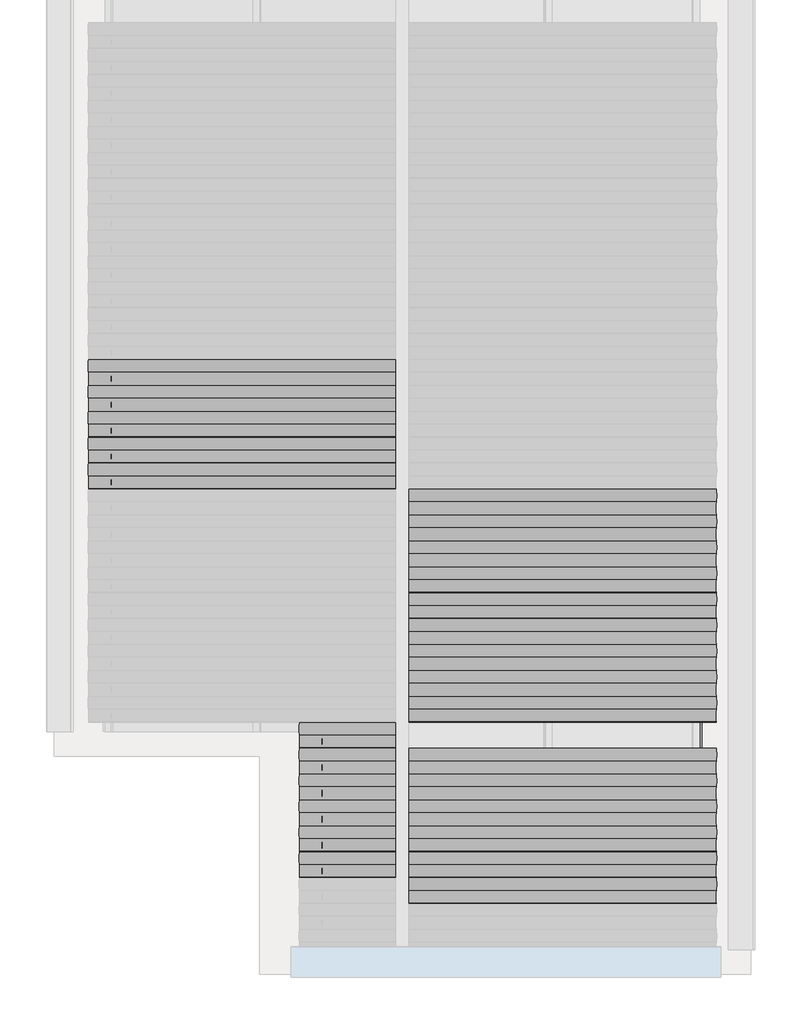
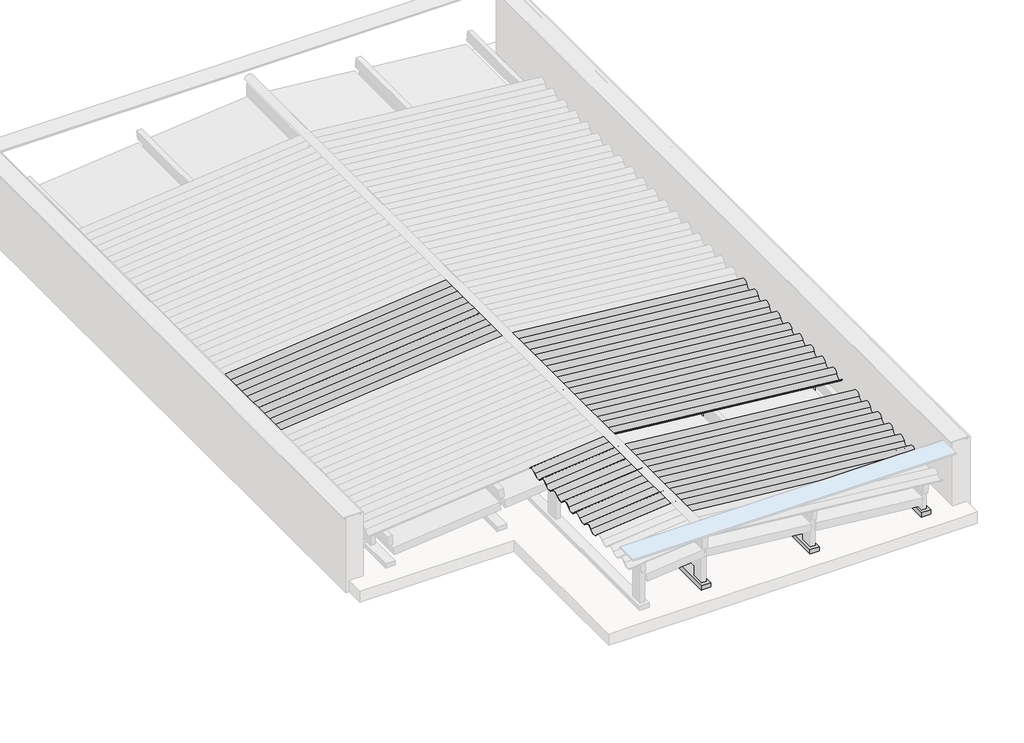
# One storey, part 2 of 4: 33 beams, 5 columns.
"""IFC4 building model written with IfcOpenShell, lengths in millimetres."""

import ifcopenshell
import ifcopenshell.guid

model = None  # the IFC model being written
_history = None  # IfcOwnerHistory: only IFC2X3 demands one
_inside = {}  # id of a spatial element -> (the spatial element, [elements in it])
_under = {}  # id of a project, library or spatial element -> (it, [spatial elements below it])
_declared = {}  # id of a project -> (the project, [libraries it declares])
_typed = {}  # id of a type object -> (the type object, [elements of that type])
_made_of = {}  # id of a material, layer set ... -> (it, [elements and type objects made of it])


def new_model(schema):
    """Start an empty IFC model of exactly this schema.

    Asked for "IFC4X3", IfcOpenShell would pick the latest addendum, in which some entities
    have other attributes; the version numbers below select the first issue.
    IFC2X3 requires an IfcOwnerHistory on every rooted entity: one is made here for all.
    """
    global model, _history
    if schema == "IFC4X3":
        model = ifcopenshell.file(schema_version=(4, 3, 0, 0))
    else:
        model = ifcopenshell.file(schema=schema)
    _inside.clear()
    _under.clear()
    _declared.clear()
    _typed.clear()
    _made_of.clear()
    _history = None
    if model.schema == "IFC2X3":
        org = make("IfcOrganization", Name="unknown")
        user = make(
            "IfcPersonAndOrganization",
            ThePerson=make("IfcPerson", FamilyName="unknown"),
            TheOrganization=org,
        )
        app = make(
            "IfcApplication",
            ApplicationDeveloper=org,
            Version="unknown",
            ApplicationFullName="unknown",
            ApplicationIdentifier="unknown",
        )
        _history = make(
            "IfcOwnerHistory",
            OwningUser=user,
            OwningApplication=app,
            ChangeAction="ADDED",
            CreationDate=0,
        )
    return model


def make(cls, **values):
    """One entity of the class cls with the attributes given. An attribute that is None is left unset."""
    return model.create_entity(
        cls, **{name: value for name, value in values.items() if value is not None}
    )


def rooted(cls, **values):
    """An entity with a GlobalId (a new one), such as an element, a storey or a relation."""
    return make(cls, GlobalId=ifcopenshell.guid.new(), OwnerHistory=_history, **values)


def si_unit(unit_type, name, prefix=None):
    """IfcSIUnit, for example si_unit("LENGTHUNIT", "METRE", prefix="MILLI")."""
    return make("IfcSIUnit", UnitType=unit_type, Prefix=prefix, Name=name)


def assignment(units):
    """IfcUnitAssignment: the units of a project."""
    return None if units is None else make("IfcUnitAssignment", Units=units)


def point(xyz):
    """IfcCartesianPoint."""
    return None if xyz is None else make("IfcCartesianPoint", Coordinates=xyz)


def direction(xyz):
    """IfcDirection."""
    return None if xyz is None else make("IfcDirection", DirectionRatios=xyz)


def frame(location, z_axis=None, x_axis=None):
    """IfcAxis2Placement3D, a coordinate frame: its origin and axes. An axis left out is left unset."""
    return make(
        "IfcAxis2Placement3D",
        Location=point(location),
        Axis=direction(z_axis),
        RefDirection=direction(x_axis),
    )


def frame_2d(location, x_axis=None):
    """IfcAxis2Placement2D, a coordinate frame in the plane: its origin and x axis."""
    return make(
        "IfcAxis2Placement2D", Location=point(location), RefDirection=direction(x_axis)
    )


def origin():
    """The frame at (0, 0, 0) with its axes left unset."""
    return frame((0.0, 0.0, 0.0))


def place(relative_to, where):
    """IfcLocalPlacement: puts the frame where relative to a parent placement (None: the world)."""
    return make(
        "IfcLocalPlacement", PlacementRelTo=relative_to, RelativePlacement=where
    )


def context(
    kind, dimensions, precision=None, world=None, true_north=None, identifier=None
):
    """IfcGeometricRepresentationContext, for example the 3D "Model" context."""
    return make(
        "IfcGeometricRepresentationContext",
        ContextIdentifier=identifier,
        ContextType=kind,
        CoordinateSpaceDimension=dimensions,
        Precision=precision,
        WorldCoordinateSystem=world,
        TrueNorth=true_north,
    )


def project(units=None, contexts=None):
    """IfcProject with its units and contexts."""
    return rooted(
        "IfcProject",
        Name="project",
        RepresentationContexts=contexts,
        UnitsInContext=assignment(units),
    )


def spatial(cls, under=None, at=None, **own):
    """A site, building, storey or space (cls), placed at a placement, below another one or the project."""
    s = rooted(cls, ObjectPlacement=at, **own)
    if under is not None:
        _under.setdefault(under.id(), (under, []))[1].append(s)
    return s


def polyline(points):
    """IfcPolyline through the points."""
    return make("IfcPolyline", Points=[point(p) for p in points])


def circle_curve(where, radius):
    """IfcCircle in the frame where."""
    return make("IfcCircle", Position=where, Radius=radius)


def trimmed(basis, trim1, trim2, sense, master):
    """IfcTrimmedCurve: the piece of a basis curve between two trims."""
    return make(
        "IfcTrimmedCurve",
        BasisCurve=basis,
        Trim1=trim1,
        Trim2=trim2,
        SenseAgreement=sense,
        MasterRepresentation=master,
    )


def segment(curve, same_sense, transition):
    """IfcCompositeCurveSegment."""
    return make(
        "IfcCompositeCurveSegment",
        Transition=transition,
        SameSense=same_sense,
        ParentCurve=curve,
    )


def composite_curve(segments, self_intersect=None):
    """IfcCompositeCurve: segments joined end to end."""
    return make("IfcCompositeCurve", Segments=segments, SelfIntersect=self_intersect)


def outline(outer, holes=None, kind="AREA"):
    """IfcArbitraryClosedProfileDef: a profile drawn as a closed curve; with holes, ...WithVoids."""
    if holes is None:
        return make("IfcArbitraryClosedProfileDef", ProfileType=kind, OuterCurve=outer)
    return make(
        "IfcArbitraryProfileDefWithVoids",
        ProfileType=kind,
        OuterCurve=outer,
        InnerCurves=holes,
    )


def extrude(swept, where, along, depth):
    """IfcExtrudedAreaSolid: the profile swept, set in the frame where, extruded along a direction by depth."""
    return make(
        "IfcExtrudedAreaSolid",
        SweptArea=swept,
        Position=where,
        ExtrudedDirection=direction(along),
        Depth=depth,
    )


def shape(context_of_items, identifier, shape_type, items):
    """IfcShapeRepresentation: the items that make up one representation, for example the "Body"."""
    return make(
        "IfcShapeRepresentation",
        ContextOfItems=context_of_items,
        RepresentationIdentifier=identifier,
        RepresentationType=shape_type,
        Items=items,
    )


def source(mapping_origin, context_of_items, identifier, shape_type, items):
    """IfcRepresentationMap: a shape defined once, which mapped items show again and again."""
    return make(
        "IfcRepresentationMap",
        MappingOrigin=mapping_origin,
        MappedRepresentation=shape(context_of_items, identifier, shape_type, items),
    )


def transform(
    local_origin,
    x_axis=None,
    y_axis=None,
    z_axis=None,
    scale=None,
    scale2=None,
    scale3=None,
    uniform=True,
):
    """IfcCartesianTransformationOperator3D, or its non-uniform kind. x_axis, y_axis, z_axis: its Axis1, 2, 3."""
    if uniform:
        return make(
            "IfcCartesianTransformationOperator3D",
            Axis1=direction(x_axis),
            Axis2=direction(y_axis),
            LocalOrigin=point(local_origin),
            Scale=scale,
            Axis3=direction(z_axis),
        )
    return make(
        "IfcCartesianTransformationOperator3DnonUniform",
        Axis1=direction(x_axis),
        Axis2=direction(y_axis),
        LocalOrigin=point(local_origin),
        Scale=scale,
        Axis3=direction(z_axis),
        Scale2=scale2,
        Scale3=scale3,
    )


def mapped(mapping_source, mapping_target):
    """IfcMappedItem: shows the shape of a source again, moved by a transform."""
    return make(
        "IfcMappedItem", MappingSource=mapping_source, MappingTarget=mapping_target
    )


def made_of(thing, what):
    """Note that an element or type object is made of a material, layer set ...; save() writes the relation."""
    if what is not None:
        _made_of.setdefault(what.id(), (what, []))[1].append(thing)
    return thing


def element(
    cls,
    number,
    at=None,
    inside=None,
    cuts=None,
    type_object=None,
    material=None,
    context=None,
    identifier="Body",
    shape_type=None,
    held_by="IfcProductDefinitionShape",
    body=None,
    shapes=None,
    **own,
):
    """One element of the class cls, such as IfcWall. Its Tag is "e" and its number.

    at: its placement. inside: the storey or other place that contains it. cuts: it is an
    opening in that element (IfcRelVoidsElement). A single representation is given by context,
    identifier, shape_type and body (its items); several are given by shapes. held_by: the class
    of the entity that holds the representations. save() writes the other relations.
    """
    e = rooted(cls, Tag="e%d" % number, ObjectPlacement=at, **own)
    if body is not None:
        shapes = [shape(context, identifier, shape_type, body)]
    if shapes is not None:
        e.Representation = make(held_by, Representations=shapes)
    if inside is not None:
        _inside.setdefault(inside.id(), (inside, []))[1].append(e)
    if cuts is not None:
        rooted(
            "IfcRelVoidsElement", RelatingBuildingElement=cuts, RelatedOpeningElement=e
        )
    if type_object is not None:
        _typed.setdefault(type_object.id(), (type_object, []))[1].append(e)
    return made_of(e, material)


def aggregate(whole, parts):
    """IfcRelAggregates: a whole, such as a stair, and the parts it consists of."""
    return rooted("IfcRelAggregates", RelatingObject=whole, RelatedObjects=parts)


def save(model, path):
    """Write the relations noted so far, then the file.

    IfcRelAggregates (storeys below a building ...), IfcRelContainedInSpatialStructure (elements
    in a storey), IfcRelDefinesByType, IfcRelAssociatesMaterial and IfcRelDeclares: one each for
    every whole, place, type object, material and project.
    """
    for whole, parts in _under.values():
        aggregate(whole, parts)
    for where, things in _inside.values():
        rooted(
            "IfcRelContainedInSpatialStructure",
            RelatedElements=things,
            RelatingStructure=where,
        )
    for kind, things in _typed.values():
        rooted("IfcRelDefinesByType", RelatedObjects=things, RelatingType=kind)
    for what, things in _made_of.values():
        rooted("IfcRelAssociatesMaterial", RelatedObjects=things, RelatingMaterial=what)
    for by, libraries in _declared.values():
        rooted("IfcRelDeclares", RelatingContext=by, RelatedDefinitions=libraries)
    model.write(path)


def column_7d6827b5(model_context):
    return source(origin(), model_context, "Body", "SweptSolid", [
        extrude(outline(polyline([(30.0, 80.0), (30.0, -80.0), (-30.0, -80.0), (-30.0, 80.0), (30.0, 80.0)])), frame((0.0, 0.0, 4460.0), z_axis=(0.0, 0.0, 1.0), x_axis=(1.0, 0.0, 0.0)), (0.0, 0.0, 1.0), 466.0),
    ])


def column_c7348c99(model_context):
    return source(origin(), model_context, "Body", "SweptSolid", [
        extrude(outline(polyline([(30.0, 80.0), (30.0, -80.0), (-30.0, -80.0), (-30.0, 80.0), (30.0, 80.0)])), frame((0.0, 0.0, 4460.0), z_axis=(0.0, 0.0, 1.0), x_axis=(1.0, 0.0, 0.0)), (0.0, 0.0, 1.0), 372.8),
    ])


def column_6cc9e01b(model_context):
    return source(origin(), model_context, "Body", "SweptSolid", [
        extrude(outline(polyline([(30.0, 80.0), (30.0, -80.0), (-30.0, -80.0), (-30.0, 80.0), (30.0, 80.0)])), frame((0.0, 0.0, 4460.0), z_axis=(0.0, 0.0, 1.0), x_axis=(1.0, 0.0, 0.0)), (0.0, 0.0, 1.0), 233.0),
    ])


model = new_model("IFC4")

# Units and contexts
model_context = context("Model", 3, world=origin())
ifc_project = project(units=[si_unit("LENGTHUNIT", "METRE", prefix="MILLI")], contexts=[model_context])

# Site, building, storey
site = spatial("IfcSite", under=ifc_project)
building = spatial("IfcBuilding", under=site)
storey = spatial("IfcBuildingStorey", under=building, Name="COB. SALA ESTAR", Elevation=4400.0)

# Beams
placement = place(None, origin())
element("IfcBeam", 1, ObjectType="Madeira de lei : Berço 6x12cm", at=placement, inside=storey, context=model_context, shape_type="SweptSolid", body=[
    extrude(outline(polyline([(-3400.8557491, 180.4300153), (-3280.8557491, 180.4300153), (-3280.8557491, -1819.5699847), (-3400.8557491, -1819.5699847), (-3400.8557491, 180.4300153)])), frame((0.0, 0.0, 4400.0), z_axis=(0.0, 0.0, 1.0), x_axis=(1.0, 0.0, 0.0)), (0.0, 0.0, 1.0), 60.0),
])
element("IfcBeam", 2, ObjectType="Madeira de lei : Berço 6x12cm", at=placement, inside=storey, context=model_context, shape_type="SweptSolid", body=[
    extrude(outline(polyline([(-3400.8557491, -1819.5699847), (-3280.8557491, -1819.5699847), (-3280.8557491, -4359.5699847), (-3400.8557491, -4359.5699847), (-3400.8557491, -1819.5699847)])), frame((0.0, 0.0, 4400.0), z_axis=(0.0, 0.0, 1.0), x_axis=(1.0, 0.0, 0.0)), (0.0, 0.0, 1.0), 60.0),
])
element("IfcBeam", 3, ObjectType="Madeira de lei : Berço 6x12cm", at=placement, inside=storey, context=model_context, shape_type="SweptSolid", body=[
    extrude(outline(polyline([(-2032.3324227, 180.4300153), (-1912.3324227, 180.4300153), (-1912.3324227, -1819.5699847), (-2032.3324227, -1819.5699847), (-2032.3324227, 180.4300153)])), frame((0.0, 0.0, 4400.0), z_axis=(0.0, 0.0, 1.0), x_axis=(1.0, 0.0, 0.0)), (0.0, 0.0, 1.0), 60.0),
])
element("IfcBeam", 4, ObjectType="Madeira de lei : Berço 6x12cm", at=placement, inside=storey, context=model_context, shape_type="SweptSolid", body=[
    extrude(outline(polyline([(-2032.3324227, -1819.5699847), (-1912.3324227, -1819.5699847), (-1912.3324227, -4359.5699847), (-2032.3324227, -4359.5699847), (-2032.3324227, -1819.5699847)])), frame((0.0, 0.0, 4400.0), z_axis=(0.0, 0.0, 1.0), x_axis=(1.0, 0.0, 0.0)), (0.0, 0.0, 1.0), 60.0),
])
element("IfcBeam", 5, ObjectType="Madeira de lei : Berço 6x12cm", at=placement, inside=storey, context=model_context, shape_type="SweptSolid", body=[
    extrude(outline(polyline([(-634.0324227, 180.4300153), (-514.0324227, 180.4300153), (-514.0324227, -1819.5699847), (-634.0324227, -1819.5699847), (-634.0324227, 180.4300153)])), frame((0.0, 0.0, 4400.0), z_axis=(0.0, 0.0, 1.0), x_axis=(1.0, 0.0, 0.0)), (0.0, 0.0, 1.0), 60.0),
])
element("IfcBeam", 6, ObjectType="Madeira de lei : Berço 6x12cm", at=placement, inside=storey, context=model_context, shape_type="SweptSolid", body=[
    extrude(outline(polyline([(-634.0324227, -1819.5699847), (-514.0324227, -1819.5699847), (-514.0324227, -4359.5699847), (-634.0324227, -4359.5699847), (-634.0324227, -1819.5699847)])), frame((0.0, 0.0, 4400.0), z_axis=(0.0, 0.0, 1.0), x_axis=(1.0, 0.0, 0.0)), (0.0, 0.0, 1.0), 60.0),
])
element("IfcBeam", 7, ObjectType="Madeira de lei : Berço 6x12cm", at=placement, inside=storey, context=model_context, shape_type="SweptSolid", body=[
    extrude(outline(polyline([(-6167.5301913, 2180.4300147), (-6047.5301913, 2180.4300147), (-6047.5301913, 180.4300153), (-6167.5301913, 180.4300153), (-6167.5301913, 2180.4300147)])), frame((0.0, 0.0, 4400.0), z_axis=(0.0, 0.0, 1.0), x_axis=(1.0, 0.0, 0.0)), (0.0, 0.0, 1.0), 60.0),
])
element("IfcBeam", 8, ObjectType="Telha Ondulada : Fibrocimento", at=placement, inside=storey, context=model_context, shape_type="SweptSolid", body=[
    extrude(outline(composite_curve([segment(trimmed(circle_curve(frame_2d((-58.7002979, -53.2060538)), 66.7939461), [point((-29.3501489, 6.7939462))], [point((-29.3501489, -113.2060538))], False, "CARTESIAN"), True, "CONTINUOUS"), segment(polyline([(-29.3501489, -113.2060538), (-31.5472155, -108.7146288)]), True, "CONTINUOUS"), segment(trimmed(circle_curve(frame_2d((-58.7002979, -53.2060538)), 61.7939461), [point((-31.5472155, -108.7146288))], [point((-31.5472155, 2.3025211))], True, "CARTESIAN"), True, "CONTINUOUS"), segment(trimmed(circle_curve(frame_2d((0.0, 66.7939462)), 71.7939461), [point((-31.5472155, 2.3025211))], [point((-31.5472155, 131.2853712))], False, "CARTESIAN"), True, "CONTINUOUS"), segment(polyline([(-31.5472155, 131.2853712), (-29.3501489, 126.7939462)]), True, "CONTINUOUS"), segment(trimmed(circle_curve(frame_2d((0.0, 66.7939462)), 66.7939461), [point((-29.3501489, 126.7939462))], [point((-29.3501489, 6.7939462))], True, "CARTESIAN"), True, "CONTINUOUS")], self_intersect=False)), frame((-4315.8870688, -3534.173052, 5061.8999542), z_axis=(0.9950371902099892, 0.0, 0.09950371902099958), x_axis=(-0.09950371902099958, 0.0, 0.9950371902099892)), (0.0, 0.0, 1.0), 970.7897678),
])
element("IfcBeam", 9, ObjectType="Telha Ondulada : Fibrocimento", at=placement, inside=storey, context=model_context, shape_type="SweptSolid", body=[
    extrude(outline(composite_curve([segment(trimmed(circle_curve(frame_2d((-58.7002979, -53.2060538)), 66.7939461), [point((-29.3501489, 6.7939462))], [point((-29.3501489, -113.2060538))], False, "CARTESIAN"), True, "CONTINUOUS"), segment(polyline([(-29.3501489, -113.2060538), (-31.5472155, -108.7146288)]), True, "CONTINUOUS"), segment(trimmed(circle_curve(frame_2d((-58.7002979, -53.2060538)), 61.7939461), [point((-31.5472155, -108.7146288))], [point((-31.5472155, 2.3025211))], True, "CARTESIAN"), True, "CONTINUOUS"), segment(trimmed(circle_curve(frame_2d((0.0, 66.7939462)), 71.7939461), [point((-31.5472155, 2.3025211))], [point((-31.5472155, 131.2853712))], False, "CARTESIAN"), True, "CONTINUOUS"), segment(polyline([(-31.5472155, 131.2853712), (-29.3501489, 126.7939462)]), True, "CONTINUOUS"), segment(trimmed(circle_curve(frame_2d((0.0, 66.7939462)), 66.7939461), [point((-29.3501489, 126.7939462))], [point((-29.3501489, 6.7939462))], True, "CARTESIAN"), True, "CONTINUOUS")], self_intersect=False)), frame((-4315.8870688, -3289.673052, 5061.8999542), z_axis=(0.9950371902099892, 0.0, 0.09950371902099958), x_axis=(-0.09950371902099958, 0.0, 0.9950371902099892)), (0.0, 0.0, 1.0), 970.7897678),
])
element("IfcBeam", 10, ObjectType="Telha Ondulada : Fibrocimento", at=placement, inside=storey, context=model_context, shape_type="SweptSolid", body=[
    extrude(outline(composite_curve([segment(trimmed(circle_curve(frame_2d((-58.7002979, -53.2060538)), 66.7939461), [point((-29.3501489, 6.7939462))], [point((-29.3501489, -113.2060538))], False, "CARTESIAN"), True, "CONTINUOUS"), segment(polyline([(-29.3501489, -113.2060538), (-31.5472155, -108.7146288)]), True, "CONTINUOUS"), segment(trimmed(circle_curve(frame_2d((-58.7002979, -53.2060538)), 61.7939461), [point((-31.5472155, -108.7146288))], [point((-31.5472155, 2.3025211))], True, "CARTESIAN"), True, "CONTINUOUS"), segment(trimmed(circle_curve(frame_2d((0.0, 66.7939462)), 71.7939461), [point((-31.5472155, 2.3025211))], [point((-31.5472155, 131.2853712))], False, "CARTESIAN"), True, "CONTINUOUS"), segment(polyline([(-31.5472155, 131.2853712), (-29.3501489, 126.7939462)]), True, "CONTINUOUS"), segment(trimmed(circle_curve(frame_2d((0.0, 66.7939462)), 66.7939461), [point((-29.3501489, 126.7939462))], [point((-29.3501489, 6.7939462))], True, "CARTESIAN"), True, "CONTINUOUS")], self_intersect=False)), frame((-4315.8870688, -3045.173052, 5061.8999542), z_axis=(0.9950371902099892, 0.0, 0.09950371902099958), x_axis=(-0.09950371902099958, 0.0, 0.9950371902099892)), (0.0, 0.0, 1.0), 970.7897678),
])
element("IfcBeam", 11, ObjectType="Telha Ondulada : Fibrocimento", at=placement, inside=storey, context=model_context, shape_type="SweptSolid", body=[
    extrude(outline(composite_curve([segment(trimmed(circle_curve(frame_2d((-58.7002979, -53.2060538)), 66.7939461), [point((-29.3501489, 6.7939462))], [point((-29.3501489, -113.2060538))], False, "CARTESIAN"), True, "CONTINUOUS"), segment(polyline([(-29.3501489, -113.2060538), (-31.5472155, -108.7146288)]), True, "CONTINUOUS"), segment(trimmed(circle_curve(frame_2d((-58.7002979, -53.2060538)), 61.7939461), [point((-31.5472155, -108.7146288))], [point((-31.5472155, 2.3025211))], True, "CARTESIAN"), True, "CONTINUOUS"), segment(trimmed(circle_curve(frame_2d((0.0, 66.7939462)), 71.7939461), [point((-31.5472155, 2.3025211))], [point((-31.5472155, 131.2853712))], False, "CARTESIAN"), True, "CONTINUOUS"), segment(polyline([(-31.5472155, 131.2853712), (-29.3501489, 126.7939462)]), True, "CONTINUOUS"), segment(trimmed(circle_curve(frame_2d((0.0, 66.7939462)), 66.7939461), [point((-29.3501489, 126.7939462))], [point((-29.3501489, 6.7939462))], True, "CARTESIAN"), True, "CONTINUOUS")], self_intersect=False)), frame((-4315.8870688, -2800.673052, 5061.8999542), z_axis=(0.9950371902099892, 0.0, 0.09950371902099964), x_axis=(-0.09950371902099964, 0.0, 0.9950371902099892)), (0.0, 0.0, 1.0), 970.7897678),
])
element("IfcBeam", 12, ObjectType="Telha Ondulada : Fibrocimento", at=placement, inside=storey, context=model_context, shape_type="SweptSolid", body=[
    extrude(outline(composite_curve([segment(trimmed(circle_curve(frame_2d((-58.7002979, -53.2060538)), 66.7939461), [point((-29.3501489, 6.7939462))], [point((-29.3501489, -113.2060538))], False, "CARTESIAN"), True, "CONTINUOUS"), segment(polyline([(-29.3501489, -113.2060538), (-31.5472155, -108.7146288)]), True, "CONTINUOUS"), segment(trimmed(circle_curve(frame_2d((-58.7002979, -53.2060538)), 61.7939461), [point((-31.5472155, -108.7146288))], [point((-31.5472155, 2.3025211))], True, "CARTESIAN"), True, "CONTINUOUS"), segment(trimmed(circle_curve(frame_2d((0.0, 66.7939462)), 71.7939461), [point((-31.5472155, 2.3025211))], [point((-31.5472155, 131.2853712))], False, "CARTESIAN"), True, "CONTINUOUS"), segment(polyline([(-31.5472155, 131.2853712), (-29.3501489, 126.7939462)]), True, "CONTINUOUS"), segment(trimmed(circle_curve(frame_2d((0.0, 66.7939462)), 66.7939461), [point((-29.3501489, 126.7939462))], [point((-29.3501489, 6.7939462))], True, "CARTESIAN"), True, "CONTINUOUS")], self_intersect=False)), frame((-4315.8870688, -2556.173052, 5061.8999542), z_axis=(0.9950371902099892, 0.0, 0.09950371902099969), x_axis=(-0.09950371902099969, 0.0, 0.9950371902099892)), (0.0, 0.0, 1.0), 970.7897678),
])
element("IfcBeam", 13, ObjectType="Telha Ondulada : Fibrocimento", at=placement, inside=storey, context=model_context, shape_type="SweptSolid", body=[
    extrude(outline(composite_curve([segment(trimmed(circle_curve(frame_2d((-58.7002979, -53.2060538)), 66.7939461), [point((-29.3501489, 6.7939462))], [point((-29.3501489, -113.2060538))], False, "CARTESIAN"), True, "CONTINUOUS"), segment(polyline([(-29.3501489, -113.2060538), (-31.5472155, -108.7146288)]), True, "CONTINUOUS"), segment(trimmed(circle_curve(frame_2d((-58.7002979, -53.2060538)), 61.7939461), [point((-31.5472155, -108.7146288))], [point((-31.5472155, 2.3025211))], True, "CARTESIAN"), True, "CONTINUOUS"), segment(trimmed(circle_curve(frame_2d((0.0, 66.7939462)), 71.7939461), [point((-31.5472155, 2.3025211))], [point((-31.5472155, 131.2853712))], False, "CARTESIAN"), True, "CONTINUOUS"), segment(polyline([(-31.5472155, 131.2853712), (-29.3501489, 126.7939462)]), True, "CONTINUOUS"), segment(trimmed(circle_curve(frame_2d((0.0, 66.7939462)), 66.7939461), [point((-29.3501489, 126.7939462))], [point((-29.3501489, 6.7939462))], True, "CARTESIAN"), True, "CONTINUOUS")], self_intersect=False)), frame((-4315.8870688, -2311.673052, 5061.8999542), z_axis=(0.9950371902099892, 0.0, 0.09950371902099958), x_axis=(-0.09950371902099958, 0.0, 0.9950371902099892)), (0.0, 0.0, 1.0), 970.7897678),
])
element("IfcBeam", 14, ObjectType="Telha Ondulada : Fibrocimento", at=placement, inside=storey, context=model_context, shape_type="SweptSolid", body=[
    extrude(outline(composite_curve([segment(trimmed(circle_curve(frame_2d((-58.7002978, -53.2060538)), 66.7939461), [point((-29.3501489, 6.7939462))], [point((-29.3501489, -113.2060538))], False, "CARTESIAN"), True, "CONTINUOUS"), segment(polyline([(-29.3501489, -113.2060538), (-31.5472154, -108.7146288)]), True, "CONTINUOUS"), segment(trimmed(circle_curve(frame_2d((-58.7002978, -53.2060538)), 61.7939461), [point((-31.5472154, -108.7146288))], [point((-31.5472154, 2.3025211))], True, "CARTESIAN"), True, "CONTINUOUS"), segment(trimmed(circle_curve(frame_2d((0.0, 66.7939462)), 71.7939461), [point((-31.5472154, 2.3025211))], [point((-31.5472154, 131.2853712))], False, "CARTESIAN"), True, "CONTINUOUS"), segment(polyline([(-31.5472154, 131.2853712), (-29.3501489, 126.7939462)]), True, "CONTINUOUS"), segment(trimmed(circle_curve(frame_2d((0.0, 66.7939462)), 66.7939461), [point((-29.3501489, 126.7939462))], [point((-29.3501489, 6.7939462))], True, "CARTESIAN"), True, "CONTINUOUS")], self_intersect=False)), frame((-6307.6707245, 133.326948, 4862.7215886), z_axis=(0.9950371902099892, 0.0, 0.09950371902099972), x_axis=(-0.09950371902099972, 0.0, 0.9950371902099892)), (0.0, 0.0, 1.0), 2972.5075682),
])
element("IfcBeam", 15, ObjectType="Telha Ondulada : Fibrocimento", at=placement, inside=storey, context=model_context, shape_type="SweptSolid", body=[
    extrude(outline(composite_curve([segment(trimmed(circle_curve(frame_2d((-58.7002978, -53.2060538)), 66.7939461), [point((-29.3501489, 6.7939462))], [point((-29.3501489, -113.2060538))], False, "CARTESIAN"), True, "CONTINUOUS"), segment(polyline([(-29.3501489, -113.2060538), (-31.5472154, -108.7146288)]), True, "CONTINUOUS"), segment(trimmed(circle_curve(frame_2d((-58.7002978, -53.2060538)), 61.7939461), [point((-31.5472154, -108.7146288))], [point((-31.5472154, 2.3025211))], True, "CARTESIAN"), True, "CONTINUOUS"), segment(trimmed(circle_curve(frame_2d((0.0, 66.7939462)), 71.7939461), [point((-31.5472154, 2.3025211))], [point((-31.5472154, 131.2853712))], False, "CARTESIAN"), True, "CONTINUOUS"), segment(polyline([(-31.5472154, 131.2853712), (-29.3501489, 126.7939462)]), True, "CONTINUOUS"), segment(trimmed(circle_curve(frame_2d((0.0, 66.7939462)), 66.7939461), [point((-29.3501489, 126.7939462))], [point((-29.3501489, 6.7939462))], True, "CARTESIAN"), True, "CONTINUOUS")], self_intersect=False)), frame((-6307.6707245, 377.826948, 4862.7215886), z_axis=(0.9950371902099892, 0.0, 0.09950371902099972), x_axis=(-0.09950371902099972, 0.0, 0.9950371902099892)), (0.0, 0.0, 1.0), 2972.5075682),
])
element("IfcBeam", 16, ObjectType="Telha Ondulada : Fibrocimento", at=placement, inside=storey, context=model_context, shape_type="SweptSolid", body=[
    extrude(outline(composite_curve([segment(trimmed(circle_curve(frame_2d((-58.7002978, -53.2060538)), 66.7939461), [point((-29.3501489, 6.7939462))], [point((-29.3501489, -113.2060538))], False, "CARTESIAN"), True, "CONTINUOUS"), segment(polyline([(-29.3501489, -113.2060538), (-31.5472154, -108.7146288)]), True, "CONTINUOUS"), segment(trimmed(circle_curve(frame_2d((-58.7002978, -53.2060538)), 61.7939461), [point((-31.5472154, -108.7146288))], [point((-31.5472154, 2.3025211))], True, "CARTESIAN"), True, "CONTINUOUS"), segment(trimmed(circle_curve(frame_2d((0.0, 66.7939462)), 71.7939461), [point((-31.5472154, 2.3025211))], [point((-31.5472154, 131.2853712))], False, "CARTESIAN"), True, "CONTINUOUS"), segment(polyline([(-31.5472154, 131.2853712), (-29.3501489, 126.7939462)]), True, "CONTINUOUS"), segment(trimmed(circle_curve(frame_2d((0.0, 66.7939462)), 66.7939461), [point((-29.3501489, 126.7939462))], [point((-29.3501489, 6.7939462))], True, "CARTESIAN"), True, "CONTINUOUS")], self_intersect=False)), frame((-6307.6707245, 622.326948, 4862.7215886), z_axis=(0.9950371902099892, 0.0, 0.09950371902099972), x_axis=(-0.09950371902099972, 0.0, 0.9950371902099892)), (0.0, 0.0, 1.0), 2972.5075682),
])
element("IfcBeam", 17, ObjectType="Telha Ondulada : Fibrocimento", at=placement, inside=storey, context=model_context, shape_type="SweptSolid", body=[
    extrude(outline(composite_curve([segment(trimmed(circle_curve(frame_2d((-58.7002978, -53.2060538)), 66.7939461), [point((-29.3501489, 6.7939462))], [point((-29.3501489, -113.2060538))], False, "CARTESIAN"), True, "CONTINUOUS"), segment(polyline([(-29.3501489, -113.2060538), (-31.5472154, -108.7146288)]), True, "CONTINUOUS"), segment(trimmed(circle_curve(frame_2d((-58.7002978, -53.2060538)), 61.7939461), [point((-31.5472154, -108.7146288))], [point((-31.5472154, 2.3025211))], True, "CARTESIAN"), True, "CONTINUOUS"), segment(trimmed(circle_curve(frame_2d((0.0, 66.7939462)), 71.7939461), [point((-31.5472154, 2.3025211))], [point((-31.5472154, 131.2853712))], False, "CARTESIAN"), True, "CONTINUOUS"), segment(polyline([(-31.5472154, 131.2853712), (-29.3501489, 126.7939462)]), True, "CONTINUOUS"), segment(trimmed(circle_curve(frame_2d((0.0, 66.7939462)), 66.7939461), [point((-29.3501489, 126.7939462))], [point((-29.3501489, 6.7939462))], True, "CARTESIAN"), True, "CONTINUOUS")], self_intersect=False)), frame((-6307.6707245, 866.826948, 4862.7215886), z_axis=(0.9950371902099892, 0.0, 0.09950371902099968), x_axis=(-0.09950371902099968, 0.0, 0.9950371902099892)), (0.0, 0.0, 1.0), 2972.5075682),
])
element("IfcBeam", 18, ObjectType="Telha Ondulada : Fibrocimento", at=placement, inside=storey, context=model_context, shape_type="SweptSolid", body=[
    extrude(outline(composite_curve([segment(trimmed(circle_curve(frame_2d((-58.7002978, -53.2060538)), 66.7939461), [point((-29.3501489, 6.7939462))], [point((-29.3501489, -113.2060538))], False, "CARTESIAN"), True, "CONTINUOUS"), segment(polyline([(-29.3501489, -113.2060538), (-31.5472154, -108.7146288)]), True, "CONTINUOUS"), segment(trimmed(circle_curve(frame_2d((-58.7002978, -53.2060538)), 61.7939461), [point((-31.5472154, -108.7146288))], [point((-31.5472154, 2.3025211))], True, "CARTESIAN"), True, "CONTINUOUS"), segment(trimmed(circle_curve(frame_2d((0.0, 66.7939462)), 71.7939461), [point((-31.5472154, 2.3025211))], [point((-31.5472154, 131.2853712))], False, "CARTESIAN"), True, "CONTINUOUS"), segment(polyline([(-31.5472154, 131.2853712), (-29.3501489, 126.7939462)]), True, "CONTINUOUS"), segment(trimmed(circle_curve(frame_2d((0.0, 66.7939462)), 66.7939461), [point((-29.3501489, 126.7939462))], [point((-29.3501489, 6.7939462))], True, "CARTESIAN"), True, "CONTINUOUS")], self_intersect=False)), frame((-6307.6707245, 1111.326948, 4862.7215886), z_axis=(0.9950371902099892, 0.0, 0.09950371902099972), x_axis=(-0.09950371902099972, 0.0, 0.9950371902099892)), (0.0, 0.0, 1.0), 2972.5075682),
])
element("IfcBeam", 19, ObjectType="Telha Ondulada : Fibrocimento", at=placement, inside=storey, context=model_context, shape_type="SweptSolid", body=[
    extrude(outline(composite_curve([segment(trimmed(circle_curve(frame_2d((0.0, 66.7939462)), 66.7939461), [point((29.3501489, 6.7939462))], [point((29.3501489, 126.7939462))], True, "CARTESIAN"), True, "CONTINUOUS"), segment(polyline([(29.3501489, 126.7939462), (31.5472154, 131.2853712)]), True, "CONTINUOUS"), segment(trimmed(circle_curve(frame_2d((0.0, 66.7939462)), 71.7939461), [point((31.5472154, 131.2853712))], [point((31.5472154, 2.3025211))], False, "CARTESIAN"), True, "CONTINUOUS"), segment(trimmed(circle_curve(frame_2d((58.7002978, -53.2060538)), 61.7939461), [point((31.5472154, 2.3025211))], [point((31.5472154, -108.7146288))], True, "CARTESIAN"), True, "CONTINUOUS"), segment(polyline([(31.5472154, -108.7146288), (29.3501489, -113.2060538)]), True, "CONTINUOUS"), segment(trimmed(circle_curve(frame_2d((58.7002978, -53.2060538)), 66.7939461), [point((29.3501489, -113.2060538))], [point((29.3501489, 6.7939462))], False, "CARTESIAN"), True, "CONTINUOUS")], self_intersect=False)), frame((-373.8918894, -3778.673052, 4862.7215886), z_axis=(-0.9950371902099892, 0.0, 0.09950371902099943), x_axis=(-0.09950371902099943, 0.0, -0.9950371902099892)), (0.0, 0.0, 1.0), 2972.5075682),
])
element("IfcBeam", 20, ObjectType="Telha Ondulada : Fibrocimento", at=placement, inside=storey, context=model_context, shape_type="SweptSolid", body=[
    extrude(outline(composite_curve([segment(trimmed(circle_curve(frame_2d((0.0, 66.7939462)), 66.7939461), [point((29.3501489, 6.7939462))], [point((29.3501489, 126.7939462))], True, "CARTESIAN"), True, "CONTINUOUS"), segment(polyline([(29.3501489, 126.7939462), (31.5472154, 131.2853712)]), True, "CONTINUOUS"), segment(trimmed(circle_curve(frame_2d((0.0, 66.7939462)), 71.7939461), [point((31.5472154, 131.2853712))], [point((31.5472154, 2.3025211))], False, "CARTESIAN"), True, "CONTINUOUS"), segment(trimmed(circle_curve(frame_2d((58.7002978, -53.2060538)), 61.7939461), [point((31.5472154, 2.3025211))], [point((31.5472154, -108.7146288))], True, "CARTESIAN"), True, "CONTINUOUS"), segment(polyline([(31.5472154, -108.7146288), (29.3501489, -113.2060538)]), True, "CONTINUOUS"), segment(trimmed(circle_curve(frame_2d((58.7002978, -53.2060538)), 66.7939461), [point((29.3501489, -113.2060538))], [point((29.3501489, 6.7939462))], False, "CARTESIAN"), True, "CONTINUOUS")], self_intersect=False)), frame((-373.8918894, -3534.173052, 4862.7215886), z_axis=(-0.9950371902099892, 0.0, 0.09950371902099943), x_axis=(-0.09950371902099943, 0.0, -0.9950371902099892)), (0.0, 0.0, 1.0), 2972.5075682),
])
element("IfcBeam", 21, ObjectType="Telha Ondulada : Fibrocimento", at=placement, inside=storey, context=model_context, shape_type="SweptSolid", body=[
    extrude(outline(composite_curve([segment(trimmed(circle_curve(frame_2d((0.0, 66.7939462)), 66.7939461), [point((29.3501489, 6.7939462))], [point((29.3501489, 126.7939462))], True, "CARTESIAN"), True, "CONTINUOUS"), segment(polyline([(29.3501489, 126.7939462), (31.5472154, 131.2853712)]), True, "CONTINUOUS"), segment(trimmed(circle_curve(frame_2d((0.0, 66.7939462)), 71.7939461), [point((31.5472154, 131.2853712))], [point((31.5472154, 2.3025211))], False, "CARTESIAN"), True, "CONTINUOUS"), segment(trimmed(circle_curve(frame_2d((58.7002978, -53.2060538)), 61.7939461), [point((31.5472154, 2.3025211))], [point((31.5472154, -108.7146288))], True, "CARTESIAN"), True, "CONTINUOUS"), segment(polyline([(31.5472154, -108.7146288), (29.3501489, -113.2060538)]), True, "CONTINUOUS"), segment(trimmed(circle_curve(frame_2d((58.7002978, -53.2060538)), 66.7939461), [point((29.3501489, -113.2060538))], [point((29.3501489, 6.7939462))], False, "CARTESIAN"), True, "CONTINUOUS")], self_intersect=False)), frame((-373.8918894, -3289.673052, 4862.7215886), z_axis=(-0.9950371902099892, 0.0, 0.09950371902099943), x_axis=(-0.09950371902099943, 0.0, -0.9950371902099892)), (0.0, 0.0, 1.0), 2972.5075682),
])
element("IfcBeam", 22, ObjectType="Telha Ondulada : Fibrocimento", at=placement, inside=storey, context=model_context, shape_type="SweptSolid", body=[
    extrude(outline(composite_curve([segment(trimmed(circle_curve(frame_2d((0.0, 66.7939462)), 66.7939461), [point((29.3501489, 6.7939462))], [point((29.3501489, 126.7939462))], True, "CARTESIAN"), True, "CONTINUOUS"), segment(polyline([(29.3501489, 126.7939462), (31.5472154, 131.2853712)]), True, "CONTINUOUS"), segment(trimmed(circle_curve(frame_2d((0.0, 66.7939462)), 71.7939461), [point((31.5472154, 131.2853712))], [point((31.5472154, 2.3025211))], False, "CARTESIAN"), True, "CONTINUOUS"), segment(trimmed(circle_curve(frame_2d((58.7002978, -53.2060538)), 61.7939461), [point((31.5472154, 2.3025211))], [point((31.5472154, -108.7146288))], True, "CARTESIAN"), True, "CONTINUOUS"), segment(polyline([(31.5472154, -108.7146288), (29.3501489, -113.2060538)]), True, "CONTINUOUS"), segment(trimmed(circle_curve(frame_2d((58.7002978, -53.2060538)), 66.7939461), [point((29.3501489, -113.2060538))], [point((29.3501489, 6.7939462))], False, "CARTESIAN"), True, "CONTINUOUS")], self_intersect=False)), frame((-373.8918894, -3045.173052, 4862.7215886), z_axis=(-0.9950371902099892, 0.0, 0.09950371902099943), x_axis=(-0.09950371902099943, 0.0, -0.9950371902099892)), (0.0, 0.0, 1.0), 2972.5075682),
])
element("IfcBeam", 23, ObjectType="Telha Ondulada : Fibrocimento", at=placement, inside=storey, context=model_context, shape_type="SweptSolid", body=[
    extrude(outline(composite_curve([segment(trimmed(circle_curve(frame_2d((0.0, 66.7939462)), 66.7939461), [point((29.3501489, 6.7939462))], [point((29.3501489, 126.7939462))], True, "CARTESIAN"), True, "CONTINUOUS"), segment(polyline([(29.3501489, 126.7939462), (31.5472154, 131.2853712)]), True, "CONTINUOUS"), segment(trimmed(circle_curve(frame_2d((0.0, 66.7939462)), 71.7939461), [point((31.5472154, 131.2853712))], [point((31.5472154, 2.3025211))], False, "CARTESIAN"), True, "CONTINUOUS"), segment(trimmed(circle_curve(frame_2d((58.7002978, -53.2060538)), 61.7939461), [point((31.5472154, 2.3025211))], [point((31.5472154, -108.7146288))], True, "CARTESIAN"), True, "CONTINUOUS"), segment(polyline([(31.5472154, -108.7146288), (29.3501489, -113.2060538)]), True, "CONTINUOUS"), segment(trimmed(circle_curve(frame_2d((58.7002978, -53.2060538)), 66.7939461), [point((29.3501489, -113.2060538))], [point((29.3501489, 6.7939462))], False, "CARTESIAN"), True, "CONTINUOUS")], self_intersect=False)), frame((-373.8918894, -2800.673052, 4862.7215886), z_axis=(-0.9950371902099892, 0.0, 0.09950371902099943), x_axis=(-0.09950371902099943, 0.0, -0.9950371902099892)), (0.0, 0.0, 1.0), 2972.5075682),
])
element("IfcBeam", 24, ObjectType="Telha Ondulada : Fibrocimento", at=placement, inside=storey, context=model_context, shape_type="SweptSolid", body=[
    extrude(outline(composite_curve([segment(trimmed(circle_curve(frame_2d((0.0, 66.7939462)), 66.7939461), [point((29.3501489, 6.7939462))], [point((29.3501489, 126.7939462))], True, "CARTESIAN"), True, "CONTINUOUS"), segment(polyline([(29.3501489, 126.7939462), (31.5472154, 131.2853712)]), True, "CONTINUOUS"), segment(trimmed(circle_curve(frame_2d((0.0, 66.7939462)), 71.7939461), [point((31.5472154, 131.2853712))], [point((31.5472154, 2.3025211))], False, "CARTESIAN"), True, "CONTINUOUS"), segment(trimmed(circle_curve(frame_2d((58.7002978, -53.2060538)), 61.7939461), [point((31.5472154, 2.3025211))], [point((31.5472154, -108.7146288))], True, "CARTESIAN"), True, "CONTINUOUS"), segment(polyline([(31.5472154, -108.7146288), (29.3501489, -113.2060538)]), True, "CONTINUOUS"), segment(trimmed(circle_curve(frame_2d((58.7002978, -53.2060538)), 66.7939461), [point((29.3501489, -113.2060538))], [point((29.3501489, 6.7939462))], False, "CARTESIAN"), True, "CONTINUOUS")], self_intersect=False)), frame((-373.8918894, -2556.173052, 4862.7215886), z_axis=(-0.9950371902099892, 0.0, 0.09950371902099943), x_axis=(-0.09950371902099943, 0.0, -0.9950371902099892)), (0.0, 0.0, 1.0), 2972.5075682),
])
element("IfcBeam", 25, ObjectType="Telha Ondulada : Fibrocimento", at=placement, inside=storey, context=model_context, shape_type="SweptSolid", body=[
    extrude(outline(composite_curve([segment(trimmed(circle_curve(frame_2d((0.0, 66.7939462)), 66.7939461), [point((29.3501489, 6.7939462))], [point((29.3501489, 126.7939462))], True, "CARTESIAN"), True, "CONTINUOUS"), segment(polyline([(29.3501489, 126.7939462), (31.5472154, 131.2853712)]), True, "CONTINUOUS"), segment(trimmed(circle_curve(frame_2d((0.0, 66.7939462)), 71.7939461), [point((31.5472154, 131.2853712))], [point((31.5472154, 2.3025211))], False, "CARTESIAN"), True, "CONTINUOUS"), segment(trimmed(circle_curve(frame_2d((58.7002978, -53.2060538)), 61.7939461), [point((31.5472154, 2.3025211))], [point((31.5472154, -108.7146288))], True, "CARTESIAN"), True, "CONTINUOUS"), segment(polyline([(31.5472154, -108.7146288), (29.3501489, -113.2060538)]), True, "CONTINUOUS"), segment(trimmed(circle_curve(frame_2d((58.7002978, -53.2060538)), 66.7939461), [point((29.3501489, -113.2060538))], [point((29.3501489, 6.7939462))], False, "CARTESIAN"), True, "CONTINUOUS")], self_intersect=False)), frame((-373.8918894, -2067.173052, 4862.7215886), z_axis=(-0.9950371902099892, 0.0, 0.09950371902099943), x_axis=(-0.09950371902099943, 0.0, -0.9950371902099892)), (0.0, 0.0, 1.0), 2972.5075682),
])
element("IfcBeam", 26, ObjectType="Telha Ondulada : Fibrocimento", at=placement, inside=storey, context=model_context, shape_type="SweptSolid", body=[
    extrude(outline(composite_curve([segment(trimmed(circle_curve(frame_2d((0.0, 66.7939462)), 66.7939461), [point((29.3501489, 6.7939462))], [point((29.3501489, 126.7939462))], True, "CARTESIAN"), True, "CONTINUOUS"), segment(polyline([(29.3501489, 126.7939462), (31.5472154, 131.2853712)]), True, "CONTINUOUS"), segment(trimmed(circle_curve(frame_2d((0.0, 66.7939462)), 71.7939461), [point((31.5472154, 131.2853712))], [point((31.5472154, 2.3025211))], False, "CARTESIAN"), True, "CONTINUOUS"), segment(trimmed(circle_curve(frame_2d((58.7002978, -53.2060538)), 61.7939461), [point((31.5472154, 2.3025211))], [point((31.5472154, -108.7146288))], True, "CARTESIAN"), True, "CONTINUOUS"), segment(polyline([(31.5472154, -108.7146288), (29.3501489, -113.2060538)]), True, "CONTINUOUS"), segment(trimmed(circle_curve(frame_2d((58.7002978, -53.2060538)), 66.7939461), [point((29.3501489, -113.2060538))], [point((29.3501489, 6.7939462))], False, "CARTESIAN"), True, "CONTINUOUS")], self_intersect=False)), frame((-373.8918894, -1822.673052, 4862.7215886), z_axis=(-0.9950371902099892, 0.0, 0.09950371902099946), x_axis=(-0.09950371902099946, 0.0, -0.9950371902099892)), (0.0, 0.0, 1.0), 2972.5075682),
])
element("IfcBeam", 27, ObjectType="Telha Ondulada : Fibrocimento", at=placement, inside=storey, context=model_context, shape_type="SweptSolid", body=[
    extrude(outline(composite_curve([segment(trimmed(circle_curve(frame_2d((0.0, 66.7939462)), 66.7939461), [point((29.3501489, 6.7939462))], [point((29.3501489, 126.7939462))], True, "CARTESIAN"), True, "CONTINUOUS"), segment(polyline([(29.3501489, 126.7939462), (31.5472154, 131.2853712)]), True, "CONTINUOUS"), segment(trimmed(circle_curve(frame_2d((0.0, 66.7939462)), 71.7939461), [point((31.5472154, 131.2853712))], [point((31.5472154, 2.3025211))], False, "CARTESIAN"), True, "CONTINUOUS"), segment(trimmed(circle_curve(frame_2d((58.7002978, -53.2060538)), 61.7939461), [point((31.5472154, 2.3025211))], [point((31.5472154, -108.7146288))], True, "CARTESIAN"), True, "CONTINUOUS"), segment(polyline([(31.5472154, -108.7146288), (29.3501489, -113.2060538)]), True, "CONTINUOUS"), segment(trimmed(circle_curve(frame_2d((58.7002978, -53.2060538)), 66.7939461), [point((29.3501489, -113.2060538))], [point((29.3501489, 6.7939462))], False, "CARTESIAN"), True, "CONTINUOUS")], self_intersect=False)), frame((-373.8918894, -1578.173052, 4862.7215886), z_axis=(-0.9950371902099892, 0.0, 0.09950371902099946), x_axis=(-0.09950371902099946, 0.0, -0.9950371902099892)), (0.0, 0.0, 1.0), 2972.5075682),
])
element("IfcBeam", 28, ObjectType="Telha Ondulada : Fibrocimento", at=placement, inside=storey, context=model_context, shape_type="SweptSolid", body=[
    extrude(outline(composite_curve([segment(trimmed(circle_curve(frame_2d((0.0, 66.7939462)), 66.7939461), [point((29.3501489, 6.7939462))], [point((29.3501489, 126.7939462))], True, "CARTESIAN"), True, "CONTINUOUS"), segment(polyline([(29.3501489, 126.7939462), (31.5472154, 131.2853712)]), True, "CONTINUOUS"), segment(trimmed(circle_curve(frame_2d((0.0, 66.7939462)), 71.7939461), [point((31.5472154, 131.2853712))], [point((31.5472154, 2.3025211))], False, "CARTESIAN"), True, "CONTINUOUS"), segment(trimmed(circle_curve(frame_2d((58.7002978, -53.2060538)), 61.7939461), [point((31.5472154, 2.3025211))], [point((31.5472154, -108.7146288))], True, "CARTESIAN"), True, "CONTINUOUS"), segment(polyline([(31.5472154, -108.7146288), (29.3501489, -113.2060538)]), True, "CONTINUOUS"), segment(trimmed(circle_curve(frame_2d((58.7002978, -53.2060538)), 66.7939461), [point((29.3501489, -113.2060538))], [point((29.3501489, 6.7939462))], False, "CARTESIAN"), True, "CONTINUOUS")], self_intersect=False)), frame((-373.8918894, -1333.673052, 4862.7215886), z_axis=(-0.9950371902099892, 0.0, 0.09950371902099946), x_axis=(-0.09950371902099946, 0.0, -0.9950371902099892)), (0.0, 0.0, 1.0), 2972.5075682),
])
element("IfcBeam", 29, ObjectType="Telha Ondulada : Fibrocimento", at=placement, inside=storey, context=model_context, shape_type="SweptSolid", body=[
    extrude(outline(composite_curve([segment(trimmed(circle_curve(frame_2d((0.0, 66.7939462)), 66.7939461), [point((29.3501489, 6.7939462))], [point((29.3501489, 126.7939462))], True, "CARTESIAN"), True, "CONTINUOUS"), segment(polyline([(29.3501489, 126.7939462), (31.5472154, 131.2853712)]), True, "CONTINUOUS"), segment(trimmed(circle_curve(frame_2d((0.0, 66.7939462)), 71.7939461), [point((31.5472154, 131.2853712))], [point((31.5472154, 2.3025211))], False, "CARTESIAN"), True, "CONTINUOUS"), segment(trimmed(circle_curve(frame_2d((58.7002978, -53.2060538)), 61.7939461), [point((31.5472154, 2.3025211))], [point((31.5472154, -108.7146288))], True, "CARTESIAN"), True, "CONTINUOUS"), segment(polyline([(31.5472154, -108.7146288), (29.3501489, -113.2060538)]), True, "CONTINUOUS"), segment(trimmed(circle_curve(frame_2d((58.7002978, -53.2060538)), 66.7939461), [point((29.3501489, -113.2060538))], [point((29.3501489, 6.7939462))], False, "CARTESIAN"), True, "CONTINUOUS")], self_intersect=False)), frame((-373.8918894, -1089.173052, 4862.7215886), z_axis=(-0.9950371902099892, 0.0, 0.09950371902099946), x_axis=(-0.09950371902099946, 0.0, -0.9950371902099892)), (0.0, 0.0, 1.0), 2972.5075682),
])
element("IfcBeam", 30, ObjectType="Telha Ondulada : Fibrocimento", at=placement, inside=storey, context=model_context, shape_type="SweptSolid", body=[
    extrude(outline(composite_curve([segment(trimmed(circle_curve(frame_2d((0.0, 66.7939462)), 66.7939461), [point((29.3501489, 6.7939462))], [point((29.3501489, 126.7939462))], True, "CARTESIAN"), True, "CONTINUOUS"), segment(polyline([(29.3501489, 126.7939462), (31.5472154, 131.2853712)]), True, "CONTINUOUS"), segment(trimmed(circle_curve(frame_2d((0.0, 66.7939462)), 71.7939461), [point((31.5472154, 131.2853712))], [point((31.5472154, 2.3025211))], False, "CARTESIAN"), True, "CONTINUOUS"), segment(trimmed(circle_curve(frame_2d((58.7002978, -53.2060538)), 61.7939461), [point((31.5472154, 2.3025211))], [point((31.5472154, -108.7146288))], True, "CARTESIAN"), True, "CONTINUOUS"), segment(polyline([(31.5472154, -108.7146288), (29.3501489, -113.2060538)]), True, "CONTINUOUS"), segment(trimmed(circle_curve(frame_2d((58.7002978, -53.2060538)), 66.7939461), [point((29.3501489, -113.2060538))], [point((29.3501489, 6.7939462))], False, "CARTESIAN"), True, "CONTINUOUS")], self_intersect=False)), frame((-373.8918894, -844.673052, 4862.7215886), z_axis=(-0.9950371902099892, 0.0, 0.09950371902099946), x_axis=(-0.09950371902099946, 0.0, -0.9950371902099892)), (0.0, 0.0, 1.0), 2972.5075682),
])
element("IfcBeam", 31, ObjectType="Telha Ondulada : Fibrocimento", at=placement, inside=storey, context=model_context, shape_type="SweptSolid", body=[
    extrude(outline(composite_curve([segment(trimmed(circle_curve(frame_2d((0.0, 66.7939462)), 66.7939461), [point((29.3501489, 6.7939462))], [point((29.3501489, 126.7939462))], True, "CARTESIAN"), True, "CONTINUOUS"), segment(polyline([(29.3501489, 126.7939462), (31.5472154, 131.2853712)]), True, "CONTINUOUS"), segment(trimmed(circle_curve(frame_2d((0.0, 66.7939462)), 71.7939461), [point((31.5472154, 131.2853712))], [point((31.5472154, 2.3025211))], False, "CARTESIAN"), True, "CONTINUOUS"), segment(trimmed(circle_curve(frame_2d((58.7002978, -53.2060538)), 61.7939461), [point((31.5472154, 2.3025211))], [point((31.5472154, -108.7146288))], True, "CARTESIAN"), True, "CONTINUOUS"), segment(polyline([(31.5472154, -108.7146288), (29.3501489, -113.2060538)]), True, "CONTINUOUS"), segment(trimmed(circle_curve(frame_2d((58.7002978, -53.2060538)), 66.7939461), [point((29.3501489, -113.2060538))], [point((29.3501489, 6.7939462))], False, "CARTESIAN"), True, "CONTINUOUS")], self_intersect=False)), frame((-373.8918894, -600.173052, 4862.7215886), z_axis=(-0.9950371902099892, 0.0, 0.09950371902099946), x_axis=(-0.09950371902099946, 0.0, -0.9950371902099892)), (0.0, 0.0, 1.0), 2972.5075682),
])
element("IfcBeam", 32, ObjectType="Telha Ondulada : Fibrocimento", at=placement, inside=storey, context=model_context, shape_type="SweptSolid", body=[
    extrude(outline(composite_curve([segment(trimmed(circle_curve(frame_2d((0.0, 66.7939462)), 66.7939461), [point((29.3501489, 6.7939462))], [point((29.3501489, 126.7939462))], True, "CARTESIAN"), True, "CONTINUOUS"), segment(polyline([(29.3501489, 126.7939462), (31.5472154, 131.2853712)]), True, "CONTINUOUS"), segment(trimmed(circle_curve(frame_2d((0.0, 66.7939462)), 71.7939461), [point((31.5472154, 131.2853712))], [point((31.5472154, 2.3025211))], False, "CARTESIAN"), True, "CONTINUOUS"), segment(trimmed(circle_curve(frame_2d((58.7002978, -53.2060538)), 61.7939461), [point((31.5472154, 2.3025211))], [point((31.5472154, -108.7146288))], True, "CARTESIAN"), True, "CONTINUOUS"), segment(polyline([(31.5472154, -108.7146288), (29.3501489, -113.2060538)]), True, "CONTINUOUS"), segment(trimmed(circle_curve(frame_2d((58.7002978, -53.2060538)), 66.7939461), [point((29.3501489, -113.2060538))], [point((29.3501489, 6.7939462))], False, "CARTESIAN"), True, "CONTINUOUS")], self_intersect=False)), frame((-373.8918894, -355.673052, 4862.7215886), z_axis=(-0.9950371902099892, 0.0, 0.09950371902099946), x_axis=(-0.09950371902099946, 0.0, -0.9950371902099892)), (0.0, 0.0, 1.0), 2972.5075682),
])
element("IfcBeam", 33, ObjectType="Telha Ondulada : Fibrocimento", at=placement, inside=storey, context=model_context, shape_type="SweptSolid", body=[
    extrude(outline(composite_curve([segment(trimmed(circle_curve(frame_2d((0.0, 66.7939462)), 66.7939461), [point((29.3501489, 6.7939462))], [point((29.3501489, 126.7939462))], True, "CARTESIAN"), True, "CONTINUOUS"), segment(polyline([(29.3501489, 126.7939462), (31.5472154, 131.2853712)]), True, "CONTINUOUS"), segment(trimmed(circle_curve(frame_2d((0.0, 66.7939462)), 71.7939461), [point((31.5472154, 131.2853712))], [point((31.5472154, 2.3025211))], False, "CARTESIAN"), True, "CONTINUOUS"), segment(trimmed(circle_curve(frame_2d((58.7002978, -53.2060538)), 61.7939461), [point((31.5472154, 2.3025211))], [point((31.5472154, -108.7146288))], True, "CARTESIAN"), True, "CONTINUOUS"), segment(polyline([(31.5472154, -108.7146288), (29.3501489, -113.2060538)]), True, "CONTINUOUS"), segment(trimmed(circle_curve(frame_2d((58.7002978, -53.2060538)), 66.7939461), [point((29.3501489, -113.2060538))], [point((29.3501489, 6.7939462))], False, "CARTESIAN"), True, "CONTINUOUS")], self_intersect=False)), frame((-373.8918894, -111.173052, 4862.7215886), z_axis=(-0.9950371902099892, 0.0, 0.09950371902099946), x_axis=(-0.09950371902099946, 0.0, -0.9950371902099892)), (0.0, 0.0, 1.0), 2972.5075682),
])

# Columns
column_shape = column_7d6827b5(model_context)
element("IfcColumn", 34, ObjectType="Madeira de lei-Coluna : Pontalete 6X16cm", at=placement, inside=storey, context=model_context, shape_type="MappedRepresentation", body=[
    mapped(column_shape, transform((-3340.8557491, -1819.5699847, 0.0), x_axis=(1.0, 0.0, 0.0), y_axis=(0.0, 1.0, 0.0), z_axis=(0.0, 0.0, 1.0))),
])
column_2_shape = column_c7348c99(model_context)
element("IfcColumn", 35, ObjectType="Madeira de lei-Coluna : Pontalete 6X16cm", at=placement, inside=storey, context=model_context, shape_type="MappedRepresentation", body=[
    mapped(column_2_shape, transform((-1972.3324227, -1819.5699847, 0.0), x_axis=(1.0, 0.0, 0.0), y_axis=(0.0, 1.0, 0.0), z_axis=(0.0, 0.0, 1.0))),
])
element("IfcColumn", 36, ObjectType="Madeira de lei-Coluna : Pontalete 6X16cm", at=placement, inside=storey, context=model_context, shape_type="MappedRepresentation", body=[
    mapped(column_2_shape, transform((-4709.2301913, 180.4300153, 0.0), x_axis=(1.0, 0.0, 0.0), y_axis=(0.0, 1.0, 0.0), z_axis=(0.0, 0.0, 1.0))),
])
column_3_shape = column_6cc9e01b(model_context)
element("IfcColumn", 37, ObjectType="Madeira de lei-Coluna : Pontalete 6X16cm", at=placement, inside=storey, context=model_context, shape_type="MappedRepresentation", body=[
    mapped(column_3_shape, transform((-574.0324227, -1819.5699847, 0.0), x_axis=(1.0, 0.0, 0.0), y_axis=(0.0, 1.0, 0.0), z_axis=(0.0, 0.0, 1.0))),
])
element("IfcColumn", 38, ObjectType="Madeira de lei-Coluna : Pontalete 6X16cm", at=placement, inside=storey, context=model_context, shape_type="MappedRepresentation", body=[
    mapped(column_3_shape, transform((-6107.5301913, 180.4300153, 0.0), x_axis=(1.0, 0.0, 0.0), y_axis=(0.0, 1.0, 0.0), z_axis=(0.0, 0.0, 1.0))),
])

save(model, "model.ifc")

# Revit data of these elements
# Type "Madeira de lei : Berço 6x12cm"
#   A = 0.02 m²
#   Length [instance default] = 1.524 m
#   b = 0.06 m
#   d = 0.12 m
#   Structural Material [instance default] = none
#   Assembly Code = ""
# Type "Telha Ondulada : Fibrocimento"
#   Description = "TELHA ONDULADA FIBROCIMENTO"
#   Cost = 5
#   Length [instance default] = 1.524 m
#   b = 0.07 m
#   h = 0.16 m
#   Structural Material = .TELHA DE FIBROCIMENTO
#   Assembly Code = ""
# Type "Madeira de lei-Coluna : Pontalete 6X16cm"
#   A = 0.01952 m²
#   b = 0.06 m
#   d = 0.16 m
#   Structural Material [instance default] = none
#   Assembly Code = ""
# Elements 1, 3, 5, 7 (IfcBeam, "Madeira de lei : Berço 6x12cm")
#   Comments = ""
#   Uso = "TELHADOS ESTRUTURAS"
#   Compr Cmcl = 6.00 m
#   Structural Material = .MADEIRAMENTO
#   Phase Created = CC_AP
#   Materials on its faces: ".MADEIRAMENTO"
# Elements 2, 4, 6 (IfcBeam, "Madeira de lei : Berço 6x12cm")
#   Comments = ""
#   Uso = "TELHADOS ESTRUTURAS"
#   Compr Cmcl = 3.00 m
#   Structural Material = .MADEIRAMENTO
#   Phase Created = CC_AP
#   Materials on its faces: ".MADEIRAMENTO"
# Elements 8, 9, 10, 11, 12, 13, 14, 15, 16, 17, 18, 19, 20, 21, 22, 23, 24, 25, 26, 27, 28, 29, 30, 31, 32, 33 (IfcBeam, "Telha Ondulada : Fibrocimento")
#   Uso = "TELHADOS TELHAS"
#   Phase Created = CC_AP
#   Materials on its faces: ".TELHA DE FIBROCIMENTO"
# Elements 34, 37, 38 (IfcColumn, "Madeira de lei-Coluna : Pontalete 6X16cm")
#   Comments = ""
#   Uso = "TELHADOS ESTRUTURAS"
#   Compr Cmcl = 3.00 m
#   Structural Material = .MADEIRAMENTO
#   Phase Created = CC_AP
#   Materials on its faces: ".MADEIRAMENTO"
# Elements 35, 36 (IfcColumn, "Madeira de lei-Coluna : Pontalete 6X16cm")
#   Comments = ""
#   Uso = "TELHADOS ESTRUTURAS"
#   Compr Cmcl = 5.00 m
#   Structural Material = .MADEIRAMENTO
#   Phase Created = CC_AP
#   Materials on its faces: ".MADEIRAMENTO"
# Materials
#   ".TELHA DE FIBROCIMENTO": class "CC_TELHADO", colour RGB 77 77 76, transparency 0, Description = "TELHA ONDULADA FIBROCIMENTO", Cost = 0
#   ".MADEIRAMENTO": class ".CC_MADEIRAS", colour RGB 212 179 113, transparency 0, Cost = 0
